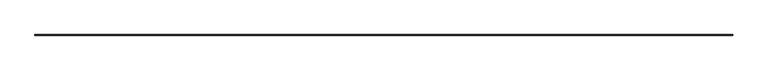
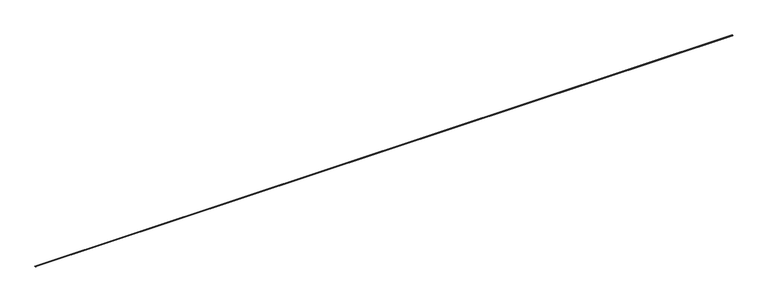
"""IFC4 building model written with IfcOpenShell, lengths in millimetres: proxy geometry, Inner panel:Inner panel:1:Inner panel:1 : Inner panel:Inner panel:300324:2:Inner panel:1:Inner panel:1 : Inner panel:Inner panel:300324:2 : Inner panel:Inner panel:1:Inner panel:1 : Inner panel:Inner panel:300324:300043:22 : Inner panel:Inner panel:1:Inner panel:1 : Inner panel:Inner panel:300324:2:Inner panel:1:Inner panel:1 : Inner panel:Inner panel:300324:2 : Inner panel:Inner panel:1:Inner panel:1 : Inner panel:Inner panel:300324:300043:308120."""

from ifc_helpers import new_model, si_unit, frame, origin, place, context, project, spatial, polyline, outline, extrude, source, transform, mapped, element, save


def generic_models_86c22ac9(model_context):
    return source(origin(), model_context, "Body", "SweptSolid", [
        extrude(outline(polyline([(-577378.0809074, 3979.3740627), (-577379.6009427, 4015.8549091), (-577422.479099, 4014.0683192), (-577420.9590637, 3977.5874729), (-577437.6334707, 3976.8927059), (-577437.7907113, 3980.6664789), (-577436.2018338, 3980.6664789), (-577436.1134355, 3978.5449182), (-577422.611276, 3979.1075081), (-577424.1313112, 4015.5883545), (-577378.0809074, 4017.5071213), (-577376.5608722, 3981.026275), (-577363.0587127, 3981.588865), (-577363.1498647, 3983.7765141), (-577361.5609873, 3983.7765141), (-577361.4065004, 3980.0688297), (-577378.0809074, 3979.3740627)])), frame((579104.5117239, 0.0, 0.0), z_axis=(1.0, 0.0, 0.0), x_axis=(0.0, 1.0, 0.0)), (0.0, 0.0, 1.0), 88442.8),
    ])


if __name__ == "__main__":
    model = new_model("IFC4")
    model_context = context("Model", 3, world=origin())
    ifc_project = project(units=[si_unit("LENGTHUNIT", "METRE", prefix="MILLI")], contexts=[model_context])
    site = spatial("IfcSite", under=ifc_project)
    building = spatial("IfcBuilding", under=site)
    placement = place(None, origin())
    generic_models_shape = generic_models_86c22ac9(model_context)
    element("IfcBuildingElementProxy", 1, Name="Inner panel:Inner panel:1:Inner panel:1 : Inner panel:Inner panel:300324:2:Inner panel:1:Inner panel:1 : Inner panel:Inner panel:300324:2 : Inner panel:Inner panel:1:Inner panel:1 : Inner panel:Inner panel:300324:300043:22 : Inner panel:Inner panel:1:Inner panel:1 : Inner panel:Inner panel:300324:2:Inner panel:1:Inner panel:1 : Inner panel:Inner panel:300324:2 : Inner panel:Inner panel:1:Inner panel:1 : Inner panel:Inner panel:300324:300043:308120", ObjectType="Inner panel:Inner panel:1:Inner panel:1 : Inner panel:Inner panel:300324:2:Inner panel:1:Inner panel:1 : Inner panel:Inner panel:300324:2 : Inner panel:Inner panel:1:Inner panel:1 : Inner panel:Inner panel:300324:300043:22 : Inner panel:Inner panel:1:Inner panel:1 : Inner panel:Inner panel:300324:2:Inner panel:1:Inner panel:1 : Inner panel:Inner panel:300324:2 : Inner panel:Inner panel:1:Inner panel:1 : Inner panel:Inner panel:300324:300043:308120", at=placement, inside=building, context=model_context, shape_type="MappedRepresentation", body=[
        mapped(generic_models_shape, transform((0.0, 0.0, 0.0), x_axis=(1.0, 0.0, 0.0), y_axis=(0.0, 1.0, 0.0), z_axis=(0.0, 0.0, 1.0))),
    ])
    save(model, "model.ifc")

# Revit data of these elements
# Type "Inner panel:Inner panel:1:Inner panel:1 : Inner panel:Inner panel:300324:2:Inner panel:1:Inner panel:1 : Inner panel:Inner panel:300324:2 : Inner panel:Inner panel:1:Inner panel:1 : Inner panel:Inner panel:300324:300043:22 : Inner panel:Inner panel:1:Inner panel:1 : Inner panel:Inner panel:300324:2:Inner panel:1:Inner panel:1 : Inner panel:Inner panel:300324:2 : Inner panel:Inner panel:1:Inner panel:1 : Inner panel:Inner panel:300324:300043:308120"
#   NameOverride = "Inner panel:Inner panel:1:Inner panel:1 : Inner panel:Inner panel:300324:2:Inner panel:1:Inner panel:1 : Inner panel:Inner panel:300324:2 : Inner panel:Inner panel:1:Inner panel:1 : Inner panel:Inner panel:300324:300043:308120"
#   ObjectTypeOverride = "Inner panel:1:Inner panel:1 : Inner panel:Inner panel:300324:2 : Inner panel:Inner panel:1:Inner panel:1 : Inner panel:Inner panel:300324:300043"
#   Reference = "Inner panel"
#   Tag = "308120"
# Element 1 (IfcBuildingElementProxy, "Inner panel:Inner panel:1:Inner panel:1 : Inner panel:Inner panel:300324:2:Inner panel:1:Inner panel:1 : Inner panel:Inner panel:300324:2 : Inner panel:Inner panel:1:Inner panel:1 : Inner panel:Inner panel:300324:300043:22 : Inner panel:Inner panel:1:Inner panel:1 : Inner panel:Inner panel:300324:2:Inner panel:1:Inner panel:1 : Inner panel:Inner panel:300324:2 : Inner panel:Inner panel:1:Inner panel:1 : Inner panel:Inner panel:300324:300043:308120")
#   Materials on its faces: "1 1/2\" HAT CHANNELS - SEE STRUCT. DWGs"
# Materials
#   "1 1/2\" HAT CHANNELS - SEE STRUCT. DWGs": class "Metal", colour RGB 189 187 185, transparency 0, Description = "Structural steel 50ksi", Cost = 0
